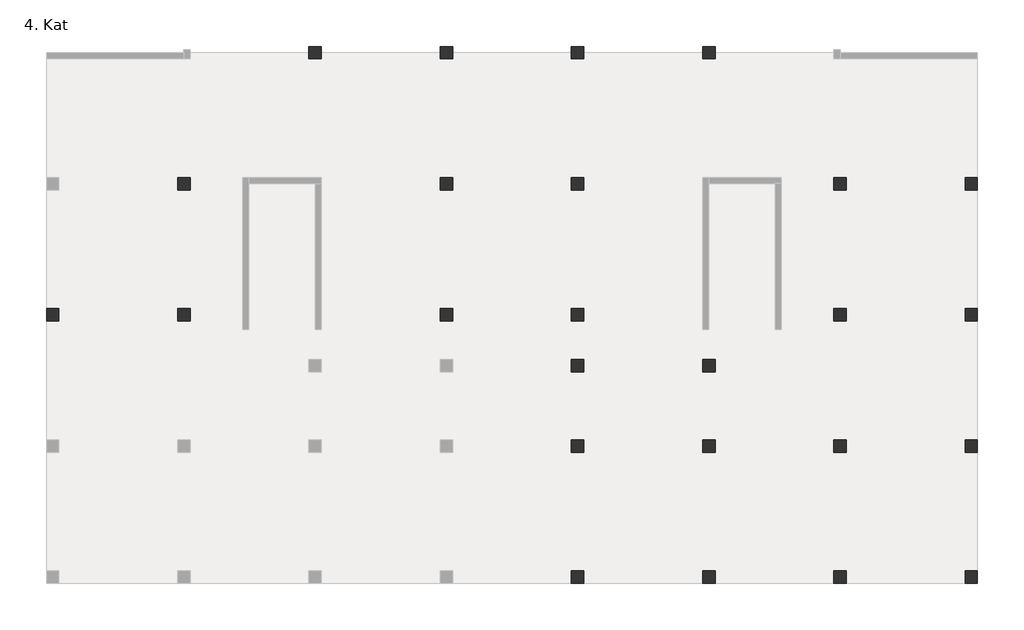
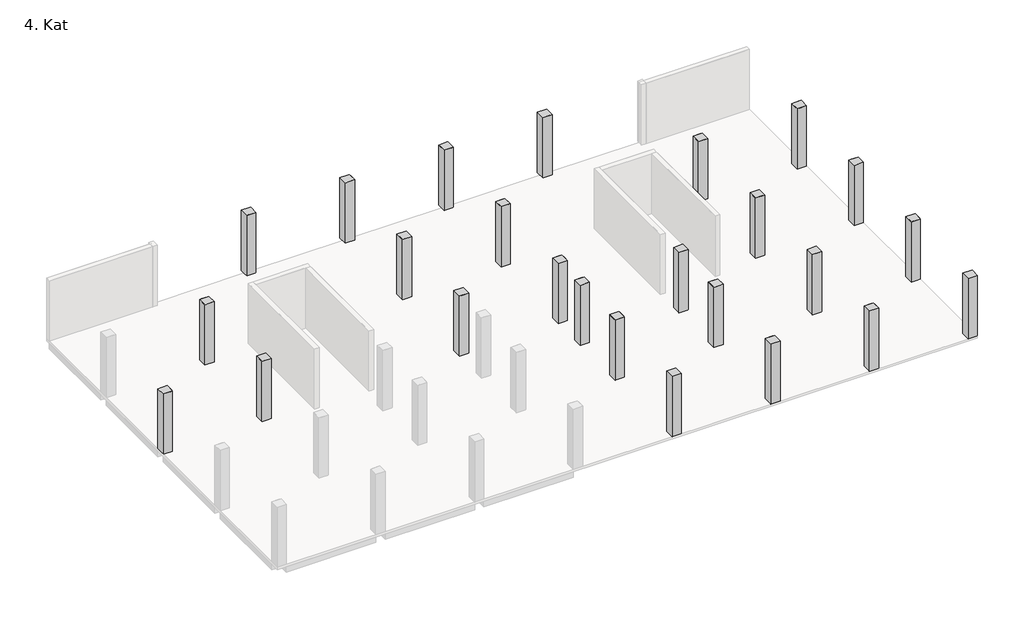
# One storey, part 2 of 2: 50 columns, 5 beams.
"""IFC4 building model written with IfcOpenShell, lengths in millimetres."""

from ifc_helpers import new_model, si_unit, frame, origin, place, context, project, spatial, polyline, outline, extrude, faceted_brep, element, save

model = new_model("IFC4")

# Units and contexts
model_context = context("Model", 3, world=origin())
ifc_project = project(units=[si_unit("LENGTHUNIT", "METRE", prefix="MILLI")], contexts=[model_context])

# Site, building, storey
site = spatial("IfcSite", under=ifc_project)
building = spatial("IfcBuilding", under=site)
storey = spatial("IfcBuildingStorey", under=building, Name="4. Kat", Elevation=21000.0)

# Beams
placement = place(None, origin())
element("IfcBeam", 1, ObjectType="M_Concrete-Rectangular Beam : 60x70cm kiriş", at=placement, inside=storey, context=model_context, shape_type="Brep", body=[
    faceted_brep([(8899.9996735, 25100.0003646, 20300.0), (8899.9996735, 25100.0003646, 20800.0), (8899.9996735, 17400.0009197, 20800.0), (8899.9996735, 17400.0009197, 20300.0), (8299.9996735, 25100.0003646, 20300.0), (8299.9996735, 17400.0009197, 20300.0), (8299.9996735, 18150.0006424, 20300.0), (8299.9996735, 18550.0006424, 20300.0), (8299.9996735, 23399.9999249, 20300.0), (8299.9996735, 23899.9999249, 20300.0), (8299.9996735, 25100.0003646, 20800.0), (8299.9996735, 17400.0009197, 20800.0), (8299.9996735, 18150.0006424, 20800.0), (8299.9996735, 18550.0006424, 20800.0), (8299.9996735, 23399.9999249, 20800.0), (8299.9996735, 23899.9999249, 20800.0)], [[[0, 1, 2, 3]], [[4, 0, 3, 5, 6, 7, 8, 9]], [[10, 4, 9, 8, 7, 6, 5, 11, 12, 13, 14, 15]], [[1, 10, 15, 14, 13, 12, 11, 2]], [[0, 4, 10, 1]], [[3, 2, 11, 5]]]),
])
element("IfcBeam", 2, ObjectType="M_Concrete-Rectangular Beam : 60x70cm kiriş", at=placement, inside=storey, context=model_context, shape_type="SweptSolid", body=[
    extrude(outline(polyline([(8899.9993907, 25899.9999188), (8299.9993907, 25899.9999188), (8299.9993907, 33600.0004302), (8899.9993907, 33600.0004302), (8899.9993907, 25899.9999188)])), frame((0.0, 0.0, 20300.0), z_axis=(0.0, 0.0, 1.0), x_axis=(1.0, 0.0, 0.0)), (0.0, 0.0, 1.0), 500.0),
])
element("IfcBeam", 3, ObjectType="M_Concrete-Rectangular Beam : 60x70cm kiriş", at=placement, inside=storey, context=model_context, shape_type="SweptSolid", body=[
    extrude(outline(polyline([(8099.9997323, 25299.999992), (399.9997323, 25299.999992), (399.9997323, 25899.999992), (8099.9997323, 25899.999992), (8099.9997323, 25299.999992)])), frame((0.0, 0.0, 20300.0), z_axis=(0.0, 0.0, 1.0), x_axis=(1.0, 0.0, 0.0)), (0.0, 0.0, 1.0), 500.0),
])
element("IfcBeam", 4, ObjectType="M_Concrete-Rectangular Beam : 50x70cm kiriş", at=placement, inside=storey, context=model_context, shape_type="SweptSolid", body=[
    extrude(outline(polyline([(199.9994072, 23399.9999249), (199.9994072, 23899.9999249), (8299.9996735, 23899.9999249), (8299.9996735, 23399.9999249), (199.9994072, 23399.9999249)])), frame((0.0, 0.0, 20300.0), z_axis=(0.0, 0.0, 1.0), x_axis=(1.0, 0.0, 0.0)), (0.0, 0.0, 1.0), 500.0),
])
element("IfcBeam", 5, ObjectType="M_Concrete-Rectangular Beam : 60x70cm kiriş", at=placement, inside=storey, context=model_context, shape_type="SweptSolid", body=[
    extrude(outline(polyline([(8099.9993907, 16800.0003638), (400.0000836, 16800.0003638), (400.0000836, 17400.0003638), (8099.9993907, 17400.0003638), (8099.9993907, 16800.0003638)])), frame((0.0, 0.0, 20300.0), z_axis=(0.0, 0.0, 1.0), x_axis=(1.0, 0.0, 0.0)), (0.0, 0.0, 1.0), 500.0),
])

# Columns
element("IfcColumn", 6, ObjectType="M_Concrete-Rectangular-Column : 80x80cm kolon", at=placement, inside=storey, context=model_context, shape_type="SweptSolid", body=[
    extrude(outline(polyline([(8899.9993907, 17400.0009197), (8899.9993907, 16600.0009197), (8099.9993907, 16600.0009197), (8099.9993907, 17400.0009197), (8899.9993907, 17400.0009197)])), frame((0.0, 0.0, 21000.0), z_axis=(0.0, 0.0, 1.0), x_axis=(1.0, 0.0, 0.0)), (0.0, 0.0, 1.0), 5500.0),
])
element("IfcColumn", 7, ObjectType="M_Concrete-Rectangular-Column : 80x80cm kolon", at=placement, inside=storey, context=model_context, shape_type="SweptSolid", body=[
    extrude(outline(polyline([(400.0000836, 17400.0009197), (400.0000836, 16600.0009197), (-399.9999164, 16600.0009197), (-399.9999164, 17400.0009197), (400.0000836, 17400.0009197)])), frame((0.0, 0.0, 21000.0), z_axis=(0.0, 0.0, 1.0), x_axis=(1.0, 0.0, 0.0)), (0.0, 0.0, 1.0), 5500.0),
])
element("IfcColumn", 8, ObjectType="M_Concrete-Rectangular-Column : 80x80cm kolon", at=placement, inside=storey, context=model_context, shape_type="SweptSolid", body=[
    extrude(outline(polyline([(8899.9993907, 25899.9999188), (8899.9993907, 25099.9999188), (8099.9993907, 25099.9999188), (8099.9993907, 25899.9999188), (8899.9993907, 25899.9999188)])), frame((0.0, 0.0, 21000.0), z_axis=(0.0, 0.0, 1.0), x_axis=(1.0, 0.0, 0.0)), (0.0, 0.0, 1.0), 5500.0),
])
element("IfcColumn", 9, ObjectType="M_Concrete-Rectangular-Column : 80x80cm kolon", at=placement, inside=storey, context=model_context, shape_type="SweptSolid", body=[
    extrude(outline(polyline([(34399.9993907, 400.0009197), (34399.9993907, -399.9990803), (33599.9993907, -399.9990803), (33599.9993907, 400.0009197), (34399.9993907, 400.0009197)])), frame((0.0, 0.0, 21000.0), z_axis=(0.0, 0.0, 1.0), x_axis=(1.0, 0.0, 0.0)), (0.0, 0.0, 1.0), 5500.0),
])
element("IfcColumn", 10, ObjectType="M_Concrete-Rectangular-Column : 80x80cm kolon", at=placement, inside=storey, context=model_context, shape_type="SweptSolid", body=[
    extrude(outline(polyline([(34399.9993907, 8900.0009197), (34399.9993907, 8100.0009197), (33599.9993907, 8100.0009197), (33599.9993907, 8900.0009197), (34399.9993907, 8900.0009197)])), frame((0.0, 0.0, 21000.0), z_axis=(0.0, 0.0, 1.0), x_axis=(1.0, 0.0, 0.0)), (0.0, 0.0, 1.0), 5500.0),
])
element("IfcColumn", 11, ObjectType="M_Concrete-Rectangular-Column : 80x80cm kolon", at=placement, inside=storey, context=model_context, shape_type="SweptSolid", body=[
    extrude(outline(polyline([(34399.9993907, 14100.0003995), (34399.9993907, 13300.0003995), (33599.9993907, 13300.0003995), (33599.9993907, 14100.0003995), (34399.9993907, 14100.0003995)])), frame((0.0, 0.0, 21000.0), z_axis=(0.0, 0.0, 1.0), x_axis=(1.0, 0.0, 0.0)), (0.0, 0.0, 1.0), 5500.0),
])
element("IfcColumn", 12, ObjectType="M_Concrete-Rectangular-Column : 80x80cm kolon", at=placement, inside=storey, context=model_context, shape_type="SweptSolid", body=[
    extrude(outline(polyline([(34399.9993907, 17400.0009197), (34399.9993907, 16600.0009197), (33599.9993907, 16600.0009197), (33599.9993907, 17400.0009197), (34399.9993907, 17400.0009197)])), frame((0.0, 0.0, 21000.0), z_axis=(0.0, 0.0, 1.0), x_axis=(1.0, 0.0, 0.0)), (0.0, 0.0, 1.0), 5500.0),
])
element("IfcColumn", 13, ObjectType="M_Concrete-Rectangular-Column : 80x80cm kolon", at=placement, inside=storey, context=model_context, shape_type="SweptSolid", body=[
    extrude(outline(polyline([(25899.9993907, 17400.0009197), (25899.9993907, 16600.0009197), (25099.9993907, 16600.0009197), (25099.9993907, 17400.0009197), (25899.9993907, 17400.0009197)])), frame((0.0, 0.0, 21000.0), z_axis=(0.0, 0.0, 1.0), x_axis=(1.0, 0.0, 0.0)), (0.0, 0.0, 1.0), 5500.0),
])
element("IfcColumn", 14, ObjectType="M_Concrete-Rectangular-Column : 80x80cm kolon", at=placement, inside=storey, context=model_context, shape_type="SweptSolid", body=[
    extrude(outline(polyline([(25899.9993907, 25900.0004105), (25899.9993907, 25100.0004105), (25099.9993907, 25100.0004105), (25099.9993907, 25900.0004105), (25899.9993907, 25900.0004105)])), frame((0.0, 0.0, 21000.0), z_axis=(0.0, 0.0, 1.0), x_axis=(1.0, 0.0, 0.0)), (0.0, 0.0, 1.0), 5500.0),
])
element("IfcColumn", 15, ObjectType="M_Concrete-Rectangular-Column : 80x80cm kolon", at=placement, inside=storey, context=model_context, shape_type="SweptSolid", body=[
    extrude(outline(polyline([(34399.9993907, 25900.0004105), (34399.9993907, 25100.0004105), (33599.9993907, 25100.0004105), (33599.9993907, 25900.0004105), (34399.9993907, 25900.0004105)])), frame((0.0, 0.0, 21000.0), z_axis=(0.0, 0.0, 1.0), x_axis=(1.0, 0.0, 0.0)), (0.0, 0.0, 1.0), 5500.0),
])
element("IfcColumn", 16, ObjectType="M_Concrete-Rectangular-Column : 80x80cm kolon", at=placement, inside=storey, context=model_context, shape_type="SweptSolid", body=[
    extrude(outline(polyline([(34399.9993907, 34400.0009197), (34399.9993907, 33600.0009197), (33599.9993907, 33600.0009197), (33599.9993907, 34400.0009197), (34399.9993907, 34400.0009197)])), frame((0.0, 0.0, 21000.0), z_axis=(0.0, 0.0, 1.0), x_axis=(1.0, 0.0, 0.0)), (0.0, 0.0, 1.0), 5500.0),
])
element("IfcColumn", 17, ObjectType="M_Concrete-Rectangular-Column : 80x80cm kolon", at=placement, inside=storey, context=model_context, shape_type="SweptSolid", body=[
    extrude(outline(polyline([(25899.9993907, 34400.0009197), (25899.9993907, 33600.0009197), (25099.9993907, 33600.0009197), (25099.9993907, 34400.0009197), (25899.9993907, 34400.0009197)])), frame((0.0, 0.0, 21000.0), z_axis=(0.0, 0.0, 1.0), x_axis=(1.0, 0.0, 0.0)), (0.0, 0.0, 1.0), 5500.0),
])
element("IfcColumn", 18, ObjectType="M_Concrete-Rectangular-Column : 80x80cm kolon", at=placement, inside=storey, context=model_context, shape_type="SweptSolid", body=[
    extrude(outline(polyline([(17399.9993907, 34400.0009197), (17399.9993907, 33600.0009197), (16599.9993907, 33600.0009197), (16599.9993907, 34400.0009197), (17399.9993907, 34400.0009197)])), frame((0.0, 0.0, 21000.0), z_axis=(0.0, 0.0, 1.0), x_axis=(1.0, 0.0, 0.0)), (0.0, 0.0, 1.0), 5500.0),
])
element("IfcColumn", 19, ObjectType="M_Concrete-Rectangular-Column : 80x80cm kolon", at=placement, inside=storey, context=model_context, shape_type="SweptSolid", body=[
    extrude(outline(polyline([(42899.9993899, 400.0009197), (42899.9993899, -399.9990803), (42099.9993899, -399.9990803), (42099.9993899, 400.0009197), (42899.9993899, 400.0009197)])), frame((0.0, 0.0, 21000.0), z_axis=(0.0, 0.0, 1.0), x_axis=(1.0, 0.0, 0.0)), (0.0, 0.0, 1.0), 5500.0),
])
element("IfcColumn", 20, ObjectType="M_Concrete-Rectangular-Column : 80x80cm kolon", at=placement, inside=storey, context=model_context, shape_type="SweptSolid", body=[
    extrude(outline(polyline([(51399.9993899, 400.0009197), (51399.9993899, -399.9990803), (50599.9993899, -399.9990803), (50599.9993899, 400.0009197), (51399.9993899, 400.0009197)])), frame((0.0, 0.0, 21000.0), z_axis=(0.0, 0.0, 1.0), x_axis=(1.0, 0.0, 0.0)), (0.0, 0.0, 1.0), 5500.0),
])
element("IfcColumn", 21, ObjectType="M_Concrete-Rectangular-Column : 80x80cm kolon", at=placement, inside=storey, context=model_context, shape_type="SweptSolid", body=[
    extrude(outline(polyline([(59900.0000836, 400.0009197), (59900.0000836, -399.9990803), (59100.0000836, -399.9990803), (59100.0000836, 400.0009197), (59900.0000836, 400.0009197)])), frame((0.0, 0.0, 21000.0), z_axis=(0.0, 0.0, 1.0), x_axis=(1.0, 0.0, 0.0)), (0.0, 0.0, 1.0), 5500.0),
])
element("IfcColumn", 22, ObjectType="M_Concrete-Rectangular-Column : 80x80cm kolon", at=placement, inside=storey, context=model_context, shape_type="SweptSolid", body=[
    extrude(outline(polyline([(59900.0000836, 8900.0009197), (59900.0000836, 8100.0009197), (59100.0000836, 8100.0009197), (59100.0000836, 8900.0009197), (59900.0000836, 8900.0009197)])), frame((0.0, 0.0, 21000.0), z_axis=(0.0, 0.0, 1.0), x_axis=(1.0, 0.0, 0.0)), (0.0, 0.0, 1.0), 5500.0),
])
element("IfcColumn", 23, ObjectType="M_Concrete-Rectangular-Column : 80x80cm kolon", at=placement, inside=storey, context=model_context, shape_type="SweptSolid", body=[
    extrude(outline(polyline([(51399.9993899, 8900.0009197), (51399.9993899, 8100.0009197), (50599.9993899, 8100.0009197), (50599.9993899, 8900.0009197), (51399.9993899, 8900.0009197)])), frame((0.0, 0.0, 21000.0), z_axis=(0.0, 0.0, 1.0), x_axis=(1.0, 0.0, 0.0)), (0.0, 0.0, 1.0), 5500.0),
])
element("IfcColumn", 24, ObjectType="M_Concrete-Rectangular-Column : 80x80cm kolon", at=placement, inside=storey, context=model_context, shape_type="SweptSolid", body=[
    extrude(outline(polyline([(42899.9993899, 8900.0009197), (42899.9993899, 8100.0009197), (42099.9993899, 8100.0009197), (42099.9993899, 8900.0009197), (42899.9993899, 8900.0009197)])), frame((0.0, 0.0, 21000.0), z_axis=(0.0, 0.0, 1.0), x_axis=(1.0, 0.0, 0.0)), (0.0, 0.0, 1.0), 5500.0),
])
element("IfcColumn", 25, ObjectType="M_Concrete-Rectangular-Column : 80x80cm kolon", at=placement, inside=storey, context=model_context, shape_type="SweptSolid", body=[
    extrude(outline(polyline([(42899.9993899, 14100.0003816), (42899.9993899, 13300.0003816), (42099.9993899, 13300.0003816), (42099.9993899, 14100.0003816), (42899.9993899, 14100.0003816)])), frame((0.0, 0.0, 21000.0), z_axis=(0.0, 0.0, 1.0), x_axis=(1.0, 0.0, 0.0)), (0.0, 0.0, 1.0), 5500.0),
])
element("IfcColumn", 26, ObjectType="M_Concrete-Rectangular-Column : 80x80cm kolon", at=placement, inside=storey, context=model_context, shape_type="SweptSolid", body=[
    extrude(outline(polyline([(51399.9993899, 17400.0009197), (51399.9993899, 16600.0009197), (50599.9993899, 16600.0009197), (50599.9993899, 17400.0009197), (51399.9993899, 17400.0009197)])), frame((0.0, 0.0, 21000.0), z_axis=(0.0, 0.0, 1.0), x_axis=(1.0, 0.0, 0.0)), (0.0, 0.0, 1.0), 5500.0),
])
element("IfcColumn", 27, ObjectType="M_Concrete-Rectangular-Column : 80x80cm kolon", at=placement, inside=storey, context=model_context, shape_type="SweptSolid", body=[
    extrude(outline(polyline([(59900.0000836, 17400.0009197), (59900.0000836, 16600.0009197), (59100.0000836, 16600.0009197), (59100.0000836, 17400.0009197), (59900.0000836, 17400.0009197)])), frame((0.0, 0.0, 21000.0), z_axis=(0.0, 0.0, 1.0), x_axis=(1.0, 0.0, 0.0)), (0.0, 0.0, 1.0), 5500.0),
])
element("IfcColumn", 28, ObjectType="M_Concrete-Rectangular-Column : 80x80cm kolon", at=placement, inside=storey, context=model_context, shape_type="SweptSolid", body=[
    extrude(outline(polyline([(51399.9993899, 25899.9999188), (51399.9993899, 25099.9999188), (50599.9993899, 25099.9999188), (50599.9993899, 25899.9999188), (51399.9993899, 25899.9999188)])), frame((0.0, 0.0, 21000.0), z_axis=(0.0, 0.0, 1.0), x_axis=(1.0, 0.0, 0.0)), (0.0, 0.0, 1.0), 5500.0),
])
element("IfcColumn", 29, ObjectType="M_Concrete-Rectangular-Column : 80x80cm kolon", at=placement, inside=storey, context=model_context, shape_type="SweptSolid", body=[
    extrude(outline(polyline([(59900.0000836, 25899.9999188), (59900.0000836, 25099.9999188), (59100.0000836, 25099.9999188), (59100.0000836, 25899.9999188), (59900.0000836, 25899.9999188)])), frame((0.0, 0.0, 21000.0), z_axis=(0.0, 0.0, 1.0), x_axis=(1.0, 0.0, 0.0)), (0.0, 0.0, 1.0), 5500.0),
])
element("IfcColumn", 30, ObjectType="M_Concrete-Rectangular-Column : 80x80cm kolon", at=placement, inside=storey, context=model_context, shape_type="SweptSolid", body=[
    extrude(outline(polyline([(42899.9993899, 34400.0009197), (42899.9993899, 33600.0009197), (42099.9993899, 33600.0009197), (42099.9993899, 34400.0009197), (42899.9993899, 34400.0009197)])), frame((0.0, 0.0, 21000.0), z_axis=(0.0, 0.0, 1.0), x_axis=(1.0, 0.0, 0.0)), (0.0, 0.0, 1.0), 5500.0),
])
element("IfcColumn", 31, ObjectType="M_Concrete-Rectangular-Column : 80x80cm kolon", at=placement, inside=storey, context=model_context, shape_type="Brep", body=[
    faceted_brep([(8899.9993907, 17400.0009197, 21000.0), (8899.9993907, 16600.0009197, 21000.0), (8099.9993907, 16600.0009197, 21000.0), (8099.9993907, 17400.0009197, 21000.0), (8899.9993907, 17400.0009197, 26500.0), (8899.9993907, 16800.0003643, 26500.0), (8899.9993907, 16600.0009197, 26500.0), (8299.9996095, 16600.0009197, 26500.0), (8099.9993907, 16600.0009197, 26500.0), (8099.9993907, 16800.0003638, 26500.0), (8099.9993907, 17400.0009197, 26500.0), (8299.9996735, 17400.0009197, 26500.0)], [[[0, 1, 2, 3]], [[4, 5, 6, 1, 0]], [[6, 7, 8, 2, 1]], [[8, 9, 10, 3, 2]], [[10, 11, 4, 0, 3]], [[4, 11, 10, 9, 8, 7, 6, 5]]]),
])
element("IfcColumn", 32, ObjectType="M_Concrete-Rectangular-Column : 80x80cm kolon", at=placement, inside=storey, context=model_context, shape_type="Brep", body=[
    faceted_brep([(400.0000836, 17400.0009197, 21000.0), (400.0000836, 16600.0009197, 21000.0), (-399.9999164, 16600.0009197, 21000.0), (-399.9999164, 17400.0009197, 21000.0), (400.0000836, 17400.0009197, 26500.0), (400.0000836, 16800.0003638, 26500.0), (400.0000836, 16600.0009197, 26500.0), (199.9996411, 16600.0009197, 26500.0), (-399.9999164, 16600.0009197, 26500.0), (-399.9999164, 17400.0009197, 26500.0), (199.9994072, 17400.0009197, 26500.0)], [[[0, 1, 2, 3]], [[4, 5, 6, 1, 0]], [[6, 7, 8, 2, 1]], [[8, 9, 3, 2]], [[9, 10, 4, 0, 3]], [[4, 10, 9, 8, 7, 6, 5]]]),
])
element("IfcColumn", 33, ObjectType="M_Concrete-Rectangular-Column : 80x80cm kolon", at=placement, inside=storey, context=model_context, shape_type="Brep", body=[
    faceted_brep([(8899.9993907, 25899.9999188, 21000.0), (8899.9993907, 25099.9999188, 21000.0), (8099.9993907, 25099.9999188, 21000.0), (8099.9993907, 25899.9999188, 21000.0), (8899.9993907, 25899.9999188, 26500.0), (8899.9993907, 25299.9999925, 26500.0), (8899.9993907, 25099.9999188, 26500.0), (8899.9993907, 25899.9999188, 25800.0), (8299.9996735, 25099.9999188, 26500.0), (8099.9993907, 25099.9999188, 26500.0), (8099.9993907, 25299.999992, 26500.0), (8099.9993907, 25899.9999188, 26500.0), (8299.9993907, 25899.9999188, 26500.0)], [[[0, 1, 2, 3]], [[4, 5, 6, 1, 0, 7]], [[6, 8, 9, 2, 1]], [[9, 10, 11, 3, 2]], [[11, 12, 4, 7, 0, 3]], [[4, 12, 11, 10, 9, 8, 6, 5]]]),
])
element("IfcColumn", 34, ObjectType="M_Concrete-Rectangular-Column : 80x80cm kolon", at=placement, inside=storey, context=model_context, shape_type="Brep", body=[
    faceted_brep([(34399.9993907, 400.0009197, 21000.0), (34399.9993907, -399.9990803, 21000.0), (33599.9993907, -399.9990803, 21000.0), (33599.9993907, 400.0009197, 21000.0), (34399.9993907, 400.0009197, 26500.0), (34399.9993907, 200.0003118, 26500.0), (34399.9993907, -399.9990803, 26500.0), (33599.9993907, -399.9990803, 26500.0), (33599.9993907, 200.0003118, 26500.0), (33599.9993907, 400.0009197, 26500.0), (34199.9997451, 400.0009197, 26500.0)], [[[0, 1, 2, 3]], [[4, 5, 6, 1, 0]], [[6, 7, 2, 1]], [[7, 8, 9, 3, 2]], [[9, 10, 4, 0, 3]], [[4, 10, 9, 8, 7, 6, 5]]]),
])
element("IfcColumn", 35, ObjectType="M_Concrete-Rectangular-Column : 80x80cm kolon", at=placement, inside=storey, context=model_context, shape_type="Brep", body=[
    faceted_brep([(34399.9993907, 8900.0009197, 21000.0), (34399.9993907, 8100.0009197, 21000.0), (33599.9993907, 8100.0009197, 21000.0), (33599.9993907, 8900.0009197, 21000.0), (34399.9993907, 8900.0009197, 26500.0), (34399.9993907, 8800.0009197, 26500.0), (34399.9993907, 8200.0009197, 26500.0), (34399.9993907, 8100.0009197, 26500.0), (34199.9997451, 8100.0009197, 26500.0), (33599.9993907, 8100.0009197, 26500.0), (33599.9993907, 8200.0009197, 26500.0), (33599.9993907, 8800.0009197, 26500.0), (33599.9993907, 8900.0009197, 26500.0), (34199.9994953, 8900.0009197, 26500.0)], [[[0, 1, 2, 3]], [[4, 5, 6, 7, 1, 0]], [[7, 8, 9, 2, 1]], [[9, 10, 11, 12, 3, 2]], [[12, 13, 4, 0, 3]], [[4, 13, 12, 11, 10, 9, 8, 7, 6, 5]]]),
])
element("IfcColumn", 36, ObjectType="M_Concrete-Rectangular-Column : 80x80cm kolon", at=placement, inside=storey, context=model_context, shape_type="Brep", body=[
    faceted_brep([(34399.9993907, 14100.0003995, 21000.0), (34399.9993907, 13300.0003995, 21000.0), (33599.9993907, 13300.0003995, 21000.0), (33599.9993907, 14100.0003995, 21000.0), (34399.9993907, 14100.0003995, 26500.0), (34399.9993907, 13700.0003995, 26500.0), (34399.9993907, 13300.0003995, 26500.0), (34399.9993907, 13300.0003995, 25800.0), (34199.9994953, 13300.0003995, 26500.0), (33599.9993907, 13300.0003995, 26500.0), (33599.9993907, 13300.0003995, 25800.0), (33599.9993907, 13700.0003995, 26500.0), (33599.9993907, 14100.0003995, 26500.0), (34199.9997451, 14100.0003995, 26500.0)], [[[0, 1, 2, 3]], [[4, 5, 6, 7, 1, 0]], [[6, 8, 9, 10, 2, 1, 7]], [[9, 11, 12, 3, 2, 10]], [[12, 13, 4, 0, 3]], [[4, 13, 12, 11, 9, 8, 6, 5]]]),
])
element("IfcColumn", 37, ObjectType="M_Concrete-Rectangular-Column : 80x80cm kolon", at=placement, inside=storey, context=model_context, shape_type="Brep", body=[
    faceted_brep([(34399.9993907, 17400.0009197, 21000.0), (34399.9993907, 16600.0009197, 21000.0), (33599.9993907, 16600.0009197, 21000.0), (33599.9993907, 17400.0009197, 21000.0), (34399.9993907, 17400.0009197, 26500.0), (34399.9993907, 17000.0007895, 26500.0), (34399.9993907, 16600.0009197, 26500.0), (34199.9997451, 16600.0009197, 26500.0), (33599.9993907, 16600.0009197, 26500.0), (33599.9993907, 17000.0007711, 26500.0), (33599.9993907, 17400.0009197, 26500.0), (34199.9994953, 17400.0009197, 26500.0)], [[[0, 1, 2, 3]], [[4, 5, 6, 1, 0]], [[6, 7, 8, 2, 1]], [[8, 9, 10, 3, 2]], [[10, 11, 4, 0, 3]], [[4, 11, 10, 9, 8, 7, 6, 5]]]),
])
element("IfcColumn", 38, ObjectType="M_Concrete-Rectangular-Column : 80x80cm kolon", at=placement, inside=storey, context=model_context, shape_type="Brep", body=[
    faceted_brep([(25899.9993907, 17400.0009197, 21000.0), (25899.9993907, 16600.0009197, 21000.0), (25099.9993907, 16600.0009197, 21000.0), (25099.9993907, 17400.0009197, 21000.0), (25899.9993907, 17400.0009197, 26500.0), (25899.9993907, 17000.0007711, 26500.0), (25899.9993907, 16600.0009197, 26500.0), (25299.9997233, 16600.0009197, 26500.0), (25099.9993907, 16600.0009197, 26500.0), (25099.9993907, 17000.0003766, 26500.0), (25099.9993907, 17400.0009197, 26500.0), (25299.999682, 17400.0009197, 26500.0)], [[[0, 1, 2, 3]], [[4, 5, 6, 1, 0]], [[6, 7, 8, 2, 1]], [[8, 9, 10, 3, 2]], [[10, 11, 4, 0, 3]], [[4, 11, 10, 9, 8, 7, 6, 5]]]),
])
element("IfcColumn", 39, ObjectType="M_Concrete-Rectangular-Column : 80x80cm kolon", at=placement, inside=storey, context=model_context, shape_type="Brep", body=[
    faceted_brep([(25899.9993907, 25900.0004105, 21000.0), (25899.9993907, 25100.0004105, 21000.0), (25099.9993907, 25100.0004105, 21000.0), (25099.9993907, 25900.0004105, 21000.0), (25899.9993907, 25900.0004105, 26500.0), (25899.9993907, 25300.0003995, 26500.0), (25899.9993907, 25100.0004105, 26500.0), (25299.999682, 25100.0004105, 26500.0), (25099.9993907, 25100.0004105, 26500.0), (25099.9993907, 25300.0000279, 26500.0), (25099.9993907, 25900.0004105, 26500.0), (25299.9996503, 25900.0004105, 26500.0)], [[[0, 1, 2, 3]], [[4, 5, 6, 1, 0]], [[6, 7, 8, 2, 1]], [[8, 9, 10, 3, 2]], [[10, 11, 4, 0, 3]], [[4, 11, 10, 9, 8, 7, 6, 5]]]),
])
element("IfcColumn", 40, ObjectType="M_Concrete-Rectangular-Column : 80x80cm kolon", at=placement, inside=storey, context=model_context, shape_type="Brep", body=[
    faceted_brep([(34399.9993907, 25900.0004105, 21000.0), (34399.9993907, 25100.0004105, 21000.0), (33599.9993907, 25100.0004105, 21000.0), (33599.9993907, 25900.0004105, 21000.0), (34399.9993907, 25900.0004105, 26500.0), (34399.9993907, 25300.0004179, 26500.0), (34399.9993907, 25100.0004105, 26500.0), (34199.9994953, 25100.0004105, 26500.0), (33599.9993907, 25100.0004105, 26500.0), (33599.9993907, 25300.0003995, 26500.0), (33599.9993907, 25900.0004105, 26500.0), (34199.9994248, 25900.0004105, 26500.0)], [[[0, 1, 2, 3]], [[4, 5, 6, 1, 0]], [[6, 7, 8, 2, 1]], [[8, 9, 10, 3, 2]], [[10, 11, 4, 0, 3]], [[4, 11, 10, 9, 8, 7, 6, 5]]]),
])
element("IfcColumn", 41, ObjectType="M_Concrete-Rectangular-Column : 80x80cm kolon", at=placement, inside=storey, context=model_context, shape_type="Brep", body=[
    faceted_brep([(34399.9993907, 34400.0009197, 21000.0), (34399.9993907, 33600.0009197, 21000.0), (33599.9993907, 33600.0009197, 21000.0), (33599.9993907, 34400.0009197, 21000.0), (34399.9993907, 34400.0009197, 26500.0), (34399.9993907, 34200.0000618, 26500.0), (34399.9993907, 33600.0009197, 26500.0), (34199.9994248, 33600.0009197, 26500.0), (33599.9993907, 33600.0009197, 26500.0), (33599.9993907, 34200.000044, 26500.0), (33599.9993907, 34400.0009197, 26500.0)], [[[0, 1, 2, 3]], [[4, 5, 6, 1, 0]], [[6, 7, 8, 2, 1]], [[8, 9, 10, 3, 2]], [[10, 4, 0, 3]], [[4, 10, 9, 8, 7, 6, 5]]]),
])
element("IfcColumn", 42, ObjectType="M_Concrete-Rectangular-Column : 80x80cm kolon", at=placement, inside=storey, context=model_context, shape_type="Brep", body=[
    faceted_brep([(25899.9993907, 34400.0009197, 21000.0), (25899.9993907, 33600.0009197, 21000.0), (25099.9993907, 33600.0009197, 21000.0), (25099.9993907, 34400.0009197, 21000.0), (25899.9993907, 34400.0009197, 26500.0), (25899.9993907, 34200.000044, 26500.0), (25899.9993907, 33600.0009197, 26500.0), (25299.9996503, 33600.0009197, 26500.0), (25099.9993907, 33600.0009197, 26500.0), (25099.9993907, 34200.0000277, 26500.0), (25099.9993907, 34400.0009197, 26500.0)], [[[0, 1, 2, 3]], [[4, 5, 6, 1, 0]], [[6, 7, 8, 2, 1]], [[8, 9, 10, 3, 2]], [[10, 4, 0, 3]], [[4, 10, 9, 8, 7, 6, 5]]]),
])
element("IfcColumn", 43, ObjectType="M_Concrete-Rectangular-Column : 80x80cm kolon", at=placement, inside=storey, context=model_context, shape_type="Brep", body=[
    faceted_brep([(17399.9993907, 34400.0009197, 21000.0), (17399.9993907, 33600.0009197, 21000.0), (16599.9993907, 33600.0009197, 21000.0), (16599.9993907, 34400.0009197, 21000.0), (17399.9993907, 34400.0009197, 26500.0), (17399.9993907, 34200.0000277, 26500.0), (17399.9993907, 33600.0009197, 26500.0), (16799.9996817, 33600.0009197, 26500.0), (16599.9993907, 33600.0009197, 26500.0), (16599.9993907, 34200.0000099, 26500.0), (16599.9993907, 34400.0009197, 26500.0)], [[[0, 1, 2, 3]], [[4, 5, 6, 1, 0]], [[6, 7, 8, 2, 1]], [[8, 9, 10, 3, 2]], [[10, 4, 0, 3]], [[4, 10, 9, 8, 7, 6, 5]]]),
])
element("IfcColumn", 44, ObjectType="M_Concrete-Rectangular-Column : 80x80cm kolon", at=placement, inside=storey, context=model_context, shape_type="Brep", body=[
    faceted_brep([(42899.9993899, 400.0009197, 21000.0), (42899.9993899, -399.9990803, 21000.0), (42099.9993899, -399.9990803, 21000.0), (42099.9993899, 400.0009197, 21000.0), (42899.9993899, 400.0009197, 26500.0), (42899.9993899, 200.0003118, 26500.0), (42899.9993899, -399.9990803, 26500.0), (42099.9993899, -399.9990803, 26500.0), (42099.9993899, 200.0003118, 26500.0), (42099.9993899, 400.0009197, 26500.0), (42699.999723, 400.0009197, 26500.0)], [[[0, 1, 2, 3]], [[4, 5, 6, 1, 0]], [[6, 7, 2, 1]], [[7, 8, 9, 3, 2]], [[9, 10, 4, 0, 3]], [[4, 10, 9, 8, 7, 6, 5]]]),
])
element("IfcColumn", 45, ObjectType="M_Concrete-Rectangular-Column : 80x80cm kolon", at=placement, inside=storey, context=model_context, shape_type="Brep", body=[
    faceted_brep([(51399.9993899, 400.0009197, 21000.0), (51399.9993899, -399.9990803, 21000.0), (50599.9993899, -399.9990803, 21000.0), (50599.9993899, 400.0009197, 21000.0), (51399.9993899, 400.0009197, 26500.0), (51399.9993899, 200.0003118, 26500.0), (51399.9993899, -399.9990803, 26500.0), (50599.9993899, -399.9990803, 26500.0), (50599.9993899, 200.0003118, 26500.0), (50599.9993899, 400.0009197, 26500.0), (51199.999723, 400.0009197, 26500.0)], [[[0, 1, 2, 3]], [[4, 5, 6, 1, 0]], [[6, 7, 2, 1]], [[7, 8, 9, 3, 2]], [[9, 10, 4, 0, 3]], [[4, 10, 9, 8, 7, 6, 5]]]),
])
element("IfcColumn", 46, ObjectType="M_Concrete-Rectangular-Column : 80x80cm kolon", at=placement, inside=storey, context=model_context, shape_type="Brep", body=[
    faceted_brep([(59900.0000836, 400.0009197, 21000.0), (59900.0000836, -399.9990803, 21000.0), (59100.0000836, -399.9990803, 21000.0), (59100.0000836, 400.0009197, 21000.0), (59900.0000836, 400.0009197, 26500.0), (59900.0000836, -399.9990803, 26500.0), (59100.0000836, -399.9990803, 26500.0), (59100.0000836, 200.0003118, 26500.0), (59100.0000836, 400.0009197, 26500.0), (59299.9997503, 400.0009197, 26500.0)], [[[0, 1, 2, 3]], [[4, 5, 1, 0]], [[5, 6, 2, 1]], [[6, 7, 8, 3, 2]], [[8, 9, 4, 0, 3]], [[4, 9, 8, 7, 6, 5]]]),
])
element("IfcColumn", 47, ObjectType="M_Concrete-Rectangular-Column : 80x80cm kolon", at=placement, inside=storey, context=model_context, shape_type="Brep", body=[
    faceted_brep([(59900.0000836, 8900.0009197, 21000.0), (59900.0000836, 8100.0009197, 21000.0), (59100.0000836, 8100.0009197, 21000.0), (59100.0000836, 8900.0009197, 21000.0), (59900.0000836, 8900.0009197, 26500.0), (59900.0000836, 8800.0009197, 26500.0), (59900.0000836, 8200.0009197, 26500.0), (59900.0000836, 8100.0009197, 26500.0), (59900.0000836, 8900.0009197, 25800.0), (59299.9997503, 8100.0009197, 26500.0), (59100.0000836, 8100.0009197, 26500.0), (59100.0000836, 8200.0009197, 26500.0), (59100.0000836, 8800.0009197, 26500.0), (59100.0000836, 8900.0009197, 26500.0), (59399.9993848, 8900.0009197, 26500.0)], [[[0, 1, 2, 3]], [[4, 5, 6, 7, 1, 0, 8]], [[7, 9, 10, 2, 1]], [[10, 11, 12, 13, 3, 2]], [[13, 14, 4, 8, 0, 3]], [[4, 14, 13, 12, 11, 10, 9, 7, 6, 5]]]),
])
element("IfcColumn", 48, ObjectType="M_Concrete-Rectangular-Column : 80x80cm kolon", at=placement, inside=storey, context=model_context, shape_type="Brep", body=[
    faceted_brep([(51399.9993899, 8900.0009197, 21000.0), (51399.9993899, 8100.0009197, 21000.0), (50599.9993899, 8100.0009197, 21000.0), (50599.9993899, 8900.0009197, 21000.0), (51399.9993899, 8900.0009197, 26500.0), (51399.9993899, 8800.0009197, 26500.0), (51399.9993899, 8200.0009197, 26500.0), (51399.9993899, 8100.0009197, 26500.0), (51199.999723, 8100.0009197, 26500.0), (50599.9993899, 8100.0009197, 26500.0), (50599.9993899, 8200.0009197, 26500.0), (50599.9993899, 8800.0009197, 26500.0), (50599.9993899, 8900.0009197, 26500.0), (51199.9996909, 8900.0009197, 26500.0)], [[[0, 1, 2, 3]], [[4, 5, 6, 7, 1, 0]], [[7, 8, 9, 2, 1]], [[9, 10, 11, 12, 3, 2]], [[12, 13, 4, 0, 3]], [[4, 13, 12, 11, 10, 9, 8, 7, 6, 5]]]),
])
element("IfcColumn", 49, ObjectType="M_Concrete-Rectangular-Column : 80x80cm kolon", at=placement, inside=storey, context=model_context, shape_type="Brep", body=[
    faceted_brep([(42899.9993899, 8900.0009197, 21000.0), (42899.9993899, 8100.0009197, 21000.0), (42099.9993899, 8100.0009197, 21000.0), (42099.9993899, 8900.0009197, 21000.0), (42899.9993899, 8900.0009197, 26500.0), (42899.9993899, 8800.0009197, 26500.0), (42899.9993899, 8200.0009197, 26500.0), (42899.9993899, 8100.0009197, 26500.0), (42699.999723, 8100.0009197, 26500.0), (42099.9993899, 8100.0009197, 26500.0), (42099.9993899, 8200.0009197, 26500.0), (42099.9993899, 8800.0009197, 26500.0), (42099.9993899, 8900.0009197, 26500.0), (42099.9993899, 8900.0009197, 25800.0), (42599.9997966, 8900.0009197, 26500.0)], [[[0, 1, 2, 3]], [[4, 5, 6, 7, 1, 0]], [[7, 8, 9, 2, 1]], [[9, 10, 11, 12, 13, 3, 2]], [[12, 14, 4, 0, 3, 13]], [[4, 14, 12, 11, 10, 9, 8, 7, 6, 5]]]),
])
element("IfcColumn", 50, ObjectType="M_Concrete-Rectangular-Column : 80x80cm kolon", at=placement, inside=storey, context=model_context, shape_type="Brep", body=[
    faceted_brep([(42899.9993899, 14100.0003816, 21000.0), (42899.9993899, 13300.0003816, 21000.0), (42099.9993899, 13300.0003816, 21000.0), (42099.9993899, 14100.0003816, 21000.0), (42899.9993899, 14100.0003816, 26500.0), (42899.9993899, 13700.0003995, 26500.0), (42899.9993899, 13300.0003816, 26500.0), (42599.9997966, 13300.0003816, 26500.0), (42099.9993899, 13300.0003816, 26500.0), (42099.9993899, 13300.0003816, 25800.0), (42099.9993899, 13700.0003995, 26500.0), (42099.9993899, 14100.0003816, 26500.0), (42499.9995162, 14100.0003816, 26500.0)], [[[0, 1, 2, 3]], [[4, 5, 6, 1, 0]], [[6, 7, 8, 9, 2, 1]], [[8, 10, 11, 3, 2, 9]], [[11, 12, 4, 0, 3]], [[4, 12, 11, 10, 8, 7, 6, 5]]]),
])
element("IfcColumn", 51, ObjectType="M_Concrete-Rectangular-Column : 80x80cm kolon", at=placement, inside=storey, context=model_context, shape_type="Brep", body=[
    faceted_brep([(51399.9993899, 17400.0009197, 21000.0), (51399.9993899, 16600.0009197, 21000.0), (50599.9993899, 16600.0009197, 21000.0), (50599.9993899, 17400.0009197, 21000.0), (51399.9993899, 17400.0009197, 26500.0), (51399.9993899, 16799.9995872, 26500.0), (51399.9993899, 16600.0009197, 26500.0), (51199.9996909, 16600.0009197, 26500.0), (50599.9993899, 16600.0009197, 26500.0), (50599.9993899, 16800.0008288, 26500.0), (50599.9993899, 17400.0009197, 26500.0), (51199.999688, 17400.0009197, 26500.0)], [[[0, 1, 2, 3]], [[4, 5, 6, 1, 0]], [[6, 7, 8, 2, 1]], [[8, 9, 10, 3, 2]], [[10, 11, 4, 0, 3]], [[4, 11, 10, 9, 8, 7, 6, 5]]]),
])
element("IfcColumn", 52, ObjectType="M_Concrete-Rectangular-Column : 80x80cm kolon", at=placement, inside=storey, context=model_context, shape_type="Brep", body=[
    faceted_brep([(59900.0000836, 17400.0009197, 21000.0), (59900.0000836, 16600.0009197, 21000.0), (59100.0000836, 16600.0009197, 21000.0), (59100.0000836, 17400.0009197, 21000.0), (59900.0000836, 17400.0009197, 26500.0), (59900.0000836, 17000.0009197, 26500.0), (59900.0000836, 16600.0009197, 26500.0), (59900.0000836, 16600.0009197, 25800.0), (59399.9993848, 16600.0009197, 26500.0), (59100.0000836, 16600.0009197, 26500.0), (59100.0000836, 16799.9995872, 26500.0), (59100.0000836, 17400.0009197, 26500.0), (59299.9997153, 17400.0009197, 26500.0)], [[[0, 1, 2, 3]], [[4, 5, 6, 7, 1, 0]], [[6, 8, 9, 2, 1, 7]], [[9, 10, 11, 3, 2]], [[11, 12, 4, 0, 3]], [[4, 12, 11, 10, 9, 8, 6, 5]]]),
])
element("IfcColumn", 53, ObjectType="M_Concrete-Rectangular-Column : 80x80cm kolon", at=placement, inside=storey, context=model_context, shape_type="Brep", body=[
    faceted_brep([(51399.9993899, 25899.9999188, 21000.0), (51399.9993899, 25099.9999188, 21000.0), (50599.9993899, 25099.9999188, 21000.0), (50599.9993899, 25899.9999188, 21000.0), (51399.9993899, 25899.9999188, 26500.0), (51399.9993899, 25300.0000972, 26500.0), (51399.9993899, 25099.9999188, 26500.0), (51199.999688, 25099.9999188, 26500.0), (50599.9993899, 25099.9999188, 26500.0), (50599.9993899, 25300.0004722, 26500.0), (50599.9993899, 25899.9999188, 26500.0), (51199.9994348, 25899.9999188, 26500.0)], [[[0, 1, 2, 3]], [[4, 5, 6, 1, 0]], [[6, 7, 8, 2, 1]], [[8, 9, 10, 3, 2]], [[10, 11, 4, 0, 3]], [[4, 11, 10, 9, 8, 7, 6, 5]]]),
])
element("IfcColumn", 54, ObjectType="M_Concrete-Rectangular-Column : 80x80cm kolon", at=placement, inside=storey, context=model_context, shape_type="Brep", body=[
    faceted_brep([(59900.0000836, 25899.9999188, 21000.0), (59900.0000836, 25099.9999188, 21000.0), (59100.0000836, 25099.9999188, 21000.0), (59100.0000836, 25899.9999188, 21000.0), (59900.0000836, 25899.9999188, 26500.0), (59900.0000836, 25099.9999188, 26500.0), (59299.9997153, 25099.9999188, 26500.0), (59100.0000836, 25099.9999188, 26500.0), (59100.0000836, 25300.0000972, 26500.0), (59100.0000836, 25899.9999188, 26500.0), (59299.9996867, 25899.9999188, 26500.0)], [[[0, 1, 2, 3]], [[4, 5, 1, 0]], [[5, 6, 7, 2, 1]], [[7, 8, 9, 3, 2]], [[9, 10, 4, 0, 3]], [[4, 10, 9, 8, 7, 6, 5]]]),
])
element("IfcColumn", 55, ObjectType="M_Concrete-Rectangular-Column : 80x80cm kolon", at=placement, inside=storey, context=model_context, shape_type="Brep", body=[
    faceted_brep([(42899.9993899, 34400.0009197, 21000.0), (42899.9993899, 33600.0009197, 21000.0), (42099.9993899, 33600.0009197, 21000.0), (42099.9993899, 34400.0009197, 21000.0), (42899.9993899, 34400.0009197, 26500.0), (42899.9993899, 34200.0000788, 26500.0), (42899.9993899, 33600.0009197, 26500.0), (42699.9994393, 33600.0009197, 26500.0), (42099.9993899, 33600.0009197, 26500.0), (42099.9993899, 34200.0000618, 26500.0), (42099.9993899, 34400.0009197, 26500.0)], [[[0, 1, 2, 3]], [[4, 5, 6, 1, 0]], [[6, 7, 8, 2, 1]], [[8, 9, 10, 3, 2]], [[10, 4, 0, 3]], [[4, 10, 9, 8, 7, 6, 5]]]),
])

save(model, "model.ifc")

# Revit data of these elements
# Type "M_Concrete-Rectangular Beam : 60x70cm kiriş"
#   Length [instance default] = 152.4 cm
#   b = 60 cm
#   h = 70 cm
#   Structural Material [instance default] = Concrete, Cast-in-Place gray
#   Assembly Code = ""
# Type "M_Concrete-Rectangular Beam : 50x70cm kiriş"
#   Length [instance default] = 152.4 cm
#   b = 50 cm
#   h = 70 cm
#   Structural Material [instance default] = Concrete, Cast-in-Place gray
#   Assembly Code = ""
# Type "M_Concrete-Rectangular-Column : 80x80cm kolon"
#   b = 80 cm
#   h = 80 cm
#   Structural Material [instance default] = Concrete, Cast-in-Place gray
# Elements 1, 2, 3, 5 (IfcBeam, "M_Concrete-Rectangular Beam : 60x70cm kiriş")
#   Comments = ""
#   Structural Material = Concrete, Cast-in-Place gray
#   Phase Created = New Construction
#   Materials on its faces: "Concrete, Cast-in-Place gray"
# Element 4 (IfcBeam, "M_Concrete-Rectangular Beam : 50x70cm kiriş")
#   Comments = ""
#   Structural Material = Concrete, Cast-in-Place gray
#   Phase Created = New Construction
#   Materials on its faces: "Concrete, Cast-in-Place gray"
# Elements 6, 7, 8, 9, 10, 11, 12, 13, 14, 15, 16, 17, 18, 19, 20, 21, 22, 23, 24, 25, 26, 27, 28, 29, 30, 31, 32, 33, 34, 35, 36, 37, 38, 39, 40, 41, 42, 43, 44, 45, 46, 47, 48, 49, 50, 51, 52, 53, 54, 55 (IfcColumn, "M_Concrete-Rectangular-Column : 80x80cm kolon")
#   Structural Material = Concrete, Cast-in-Place gray
#   Phase Created = New Construction
#   Materials on its faces: "Concrete, Cast-in-Place gray"
# Materials
#   "Concrete, Cast-in-Place gray": class "Concrete", colour RGB 192 192 192, transparency 0, Description = "Cast-in-place concrete", Cost = 0
